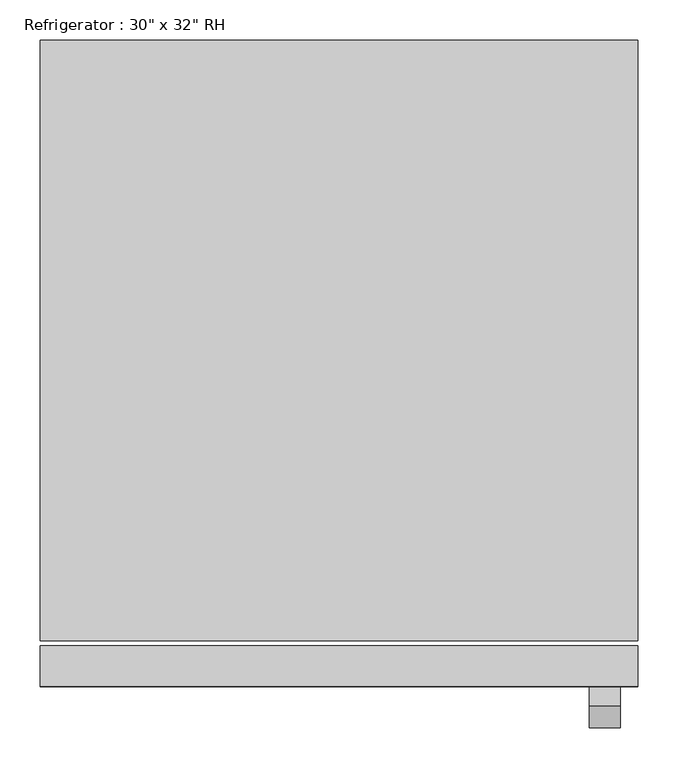
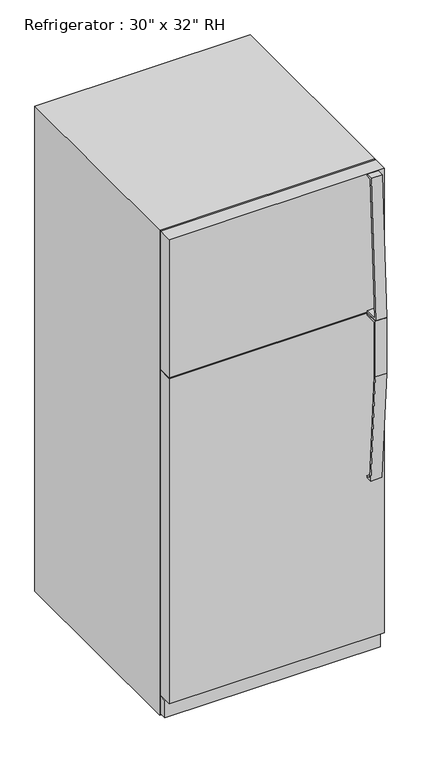
"""IFC4 building model written with IfcOpenShell, lengths in millimetres: proxy geometry."""

import ifcopenshell
import ifcopenshell.guid

model = None  # the IFC model being written
_history = None  # IfcOwnerHistory: only IFC2X3 demands one
_inside = {}  # id of a spatial element -> (the spatial element, [elements in it])
_under = {}  # id of a project, library or spatial element -> (it, [spatial elements below it])
_declared = {}  # id of a project -> (the project, [libraries it declares])
_typed = {}  # id of a type object -> (the type object, [elements of that type])
_made_of = {}  # id of a material, layer set ... -> (it, [elements and type objects made of it])


def new_model(schema):
    """Start an empty IFC model of exactly this schema.

    Asked for "IFC4X3", IfcOpenShell would pick the latest addendum, in which some entities
    have other attributes; the version numbers below select the first issue.
    IFC2X3 requires an IfcOwnerHistory on every rooted entity: one is made here for all.
    """
    global model, _history
    if schema == "IFC4X3":
        model = ifcopenshell.file(schema_version=(4, 3, 0, 0))
    else:
        model = ifcopenshell.file(schema=schema)
    _inside.clear()
    _under.clear()
    _declared.clear()
    _typed.clear()
    _made_of.clear()
    _history = None
    if model.schema == "IFC2X3":
        org = make("IfcOrganization", Name="unknown")
        user = make(
            "IfcPersonAndOrganization",
            ThePerson=make("IfcPerson", FamilyName="unknown"),
            TheOrganization=org,
        )
        app = make(
            "IfcApplication",
            ApplicationDeveloper=org,
            Version="unknown",
            ApplicationFullName="unknown",
            ApplicationIdentifier="unknown",
        )
        _history = make(
            "IfcOwnerHistory",
            OwningUser=user,
            OwningApplication=app,
            ChangeAction="ADDED",
            CreationDate=0,
        )
    return model


def make(cls, **values):
    """One entity of the class cls with the attributes given. An attribute that is None is left unset."""
    return model.create_entity(
        cls, **{name: value for name, value in values.items() if value is not None}
    )


def rooted(cls, **values):
    """An entity with a GlobalId (a new one), such as an element, a storey or a relation."""
    return make(cls, GlobalId=ifcopenshell.guid.new(), OwnerHistory=_history, **values)


def si_unit(unit_type, name, prefix=None):
    """IfcSIUnit, for example si_unit("LENGTHUNIT", "METRE", prefix="MILLI")."""
    return make("IfcSIUnit", UnitType=unit_type, Prefix=prefix, Name=name)


def assignment(units):
    """IfcUnitAssignment: the units of a project."""
    return None if units is None else make("IfcUnitAssignment", Units=units)


def point(xyz):
    """IfcCartesianPoint."""
    return None if xyz is None else make("IfcCartesianPoint", Coordinates=xyz)


def direction(xyz):
    """IfcDirection."""
    return None if xyz is None else make("IfcDirection", DirectionRatios=xyz)


def frame(location, z_axis=None, x_axis=None):
    """IfcAxis2Placement3D, a coordinate frame: its origin and axes. An axis left out is left unset."""
    return make(
        "IfcAxis2Placement3D",
        Location=point(location),
        Axis=direction(z_axis),
        RefDirection=direction(x_axis),
    )


def origin():
    """The frame at (0, 0, 0) with its axes left unset."""
    return frame((0.0, 0.0, 0.0))


def origin_with_axes():
    """The frame at (0, 0, 0) with the z axis (0, 0, 1) and the x axis (1, 0, 0) written out."""
    return frame((0.0, 0.0, 0.0), z_axis=(0.0, 0.0, 1.0), x_axis=(1.0, 0.0, 0.0))


def place(relative_to, where):
    """IfcLocalPlacement: puts the frame where relative to a parent placement (None: the world)."""
    return make(
        "IfcLocalPlacement", PlacementRelTo=relative_to, RelativePlacement=where
    )


def context(
    kind, dimensions, precision=None, world=None, true_north=None, identifier=None
):
    """IfcGeometricRepresentationContext, for example the 3D "Model" context."""
    return make(
        "IfcGeometricRepresentationContext",
        ContextIdentifier=identifier,
        ContextType=kind,
        CoordinateSpaceDimension=dimensions,
        Precision=precision,
        WorldCoordinateSystem=world,
        TrueNorth=true_north,
    )


def project(units=None, contexts=None):
    """IfcProject with its units and contexts."""
    return rooted(
        "IfcProject",
        Name="project",
        RepresentationContexts=contexts,
        UnitsInContext=assignment(units),
    )


def spatial(cls, under=None, at=None, **own):
    """A site, building, storey or space (cls), placed at a placement, below another one or the project."""
    s = rooted(cls, ObjectPlacement=at, **own)
    if under is not None:
        _under.setdefault(under.id(), (under, []))[1].append(s)
    return s


def polyline(points):
    """IfcPolyline through the points."""
    return make("IfcPolyline", Points=[point(p) for p in points])


def outline(outer, holes=None, kind="AREA"):
    """IfcArbitraryClosedProfileDef: a profile drawn as a closed curve; with holes, ...WithVoids."""
    if holes is None:
        return make("IfcArbitraryClosedProfileDef", ProfileType=kind, OuterCurve=outer)
    return make(
        "IfcArbitraryProfileDefWithVoids",
        ProfileType=kind,
        OuterCurve=outer,
        InnerCurves=holes,
    )


def extrude(swept, where, along, depth):
    """IfcExtrudedAreaSolid: the profile swept, set in the frame where, extruded along a direction by depth."""
    return make(
        "IfcExtrudedAreaSolid",
        SweptArea=swept,
        Position=where,
        ExtrudedDirection=direction(along),
        Depth=depth,
    )


def shape(context_of_items, identifier, shape_type, items):
    """IfcShapeRepresentation: the items that make up one representation, for example the "Body"."""
    return make(
        "IfcShapeRepresentation",
        ContextOfItems=context_of_items,
        RepresentationIdentifier=identifier,
        RepresentationType=shape_type,
        Items=items,
    )


def source(mapping_origin, context_of_items, identifier, shape_type, items):
    """IfcRepresentationMap: a shape defined once, which mapped items show again and again."""
    return make(
        "IfcRepresentationMap",
        MappingOrigin=mapping_origin,
        MappedRepresentation=shape(context_of_items, identifier, shape_type, items),
    )


def transform(
    local_origin,
    x_axis=None,
    y_axis=None,
    z_axis=None,
    scale=None,
    scale2=None,
    scale3=None,
    uniform=True,
):
    """IfcCartesianTransformationOperator3D, or its non-uniform kind. x_axis, y_axis, z_axis: its Axis1, 2, 3."""
    if uniform:
        return make(
            "IfcCartesianTransformationOperator3D",
            Axis1=direction(x_axis),
            Axis2=direction(y_axis),
            LocalOrigin=point(local_origin),
            Scale=scale,
            Axis3=direction(z_axis),
        )
    return make(
        "IfcCartesianTransformationOperator3DnonUniform",
        Axis1=direction(x_axis),
        Axis2=direction(y_axis),
        LocalOrigin=point(local_origin),
        Scale=scale,
        Axis3=direction(z_axis),
        Scale2=scale2,
        Scale3=scale3,
    )


def mapped(mapping_source, mapping_target):
    """IfcMappedItem: shows the shape of a source again, moved by a transform."""
    return make(
        "IfcMappedItem", MappingSource=mapping_source, MappingTarget=mapping_target
    )


def made_of(thing, what):
    """Note that an element or type object is made of a material, layer set ...; save() writes the relation."""
    if what is not None:
        _made_of.setdefault(what.id(), (what, []))[1].append(thing)
    return thing


def element(
    cls,
    number,
    at=None,
    inside=None,
    cuts=None,
    type_object=None,
    material=None,
    context=None,
    identifier="Body",
    shape_type=None,
    held_by="IfcProductDefinitionShape",
    body=None,
    shapes=None,
    **own,
):
    """One element of the class cls, such as IfcWall. Its Tag is "e" and its number.

    at: its placement. inside: the storey or other place that contains it. cuts: it is an
    opening in that element (IfcRelVoidsElement). A single representation is given by context,
    identifier, shape_type and body (its items); several are given by shapes. held_by: the class
    of the entity that holds the representations. save() writes the other relations.
    """
    e = rooted(cls, Tag="e%d" % number, ObjectPlacement=at, **own)
    if body is not None:
        shapes = [shape(context, identifier, shape_type, body)]
    if shapes is not None:
        e.Representation = make(held_by, Representations=shapes)
    if inside is not None:
        _inside.setdefault(inside.id(), (inside, []))[1].append(e)
    if cuts is not None:
        rooted(
            "IfcRelVoidsElement", RelatingBuildingElement=cuts, RelatedOpeningElement=e
        )
    if type_object is not None:
        _typed.setdefault(type_object.id(), (type_object, []))[1].append(e)
    return made_of(e, material)


def aggregate(whole, parts):
    """IfcRelAggregates: a whole, such as a stair, and the parts it consists of."""
    return rooted("IfcRelAggregates", RelatingObject=whole, RelatedObjects=parts)


def save(model, path):
    """Write the relations noted so far, then the file.

    IfcRelAggregates (storeys below a building ...), IfcRelContainedInSpatialStructure (elements
    in a storey), IfcRelDefinesByType, IfcRelAssociatesMaterial and IfcRelDeclares: one each for
    every whole, place, type object, material and project.
    """
    for whole, parts in _under.values():
        aggregate(whole, parts)
    for where, things in _inside.values():
        rooted(
            "IfcRelContainedInSpatialStructure",
            RelatedElements=things,
            RelatingStructure=where,
        )
    for kind, things in _typed.values():
        rooted("IfcRelDefinesByType", RelatedObjects=things, RelatingType=kind)
    for what, things in _made_of.values():
        rooted("IfcRelAssociatesMaterial", RelatedObjects=things, RelatingMaterial=what)
    for by, libraries in _declared.values():
        rooted("IfcRelDeclares", RelatingContext=by, RelatedDefinitions=libraries)
    model.write(path)


def proxy_a13a33b2(model_context):
    return source(origin(), model_context, "Body", "SweptSolid", [
        extrude(outline(polyline([(-417.9010285, 1262.0625), (-462.3510285, 1262.0625), (-462.3510285, 1065.4342469), (-434.8723987, 672.4715334), (-417.9010285, 672.4715334), (-417.9010285, 666.1370017), (-440.7949512, 666.1370017), (-468.7010285, 1065.2125), (-468.7010285, 1268.4125), (-417.9010285, 1268.4125), (-417.9010285, 1262.0625)])), frame((312.7375, 0.0, 0.0), z_axis=(1.0, 0.0, 0.0), x_axis=(0.0, 1.0, 0.0)), (0.0, 0.0, 1.0), 38.4332978),
        extrude(outline(polyline([(-442.739413, 1778.0), (-418.6780855, 1778.0), (-418.6780855, 1771.65), (-437.5263449, 1771.65), (-463.4007207, 1277.9375), (-418.6780855, 1277.9375), (-418.6780855, 1271.5875), (-469.2793675, 1271.5875), (-442.739413, 1778.0)])), frame((312.7375, 0.0, 0.0), z_axis=(1.0, 0.0, 0.0), x_axis=(0.0, 1.0, 0.0)), (0.0, 0.0, 1.0), 38.4332978),
        extrude(outline(polyline([(373.0625, -367.1010285), (373.0625, -392.5010285), (-373.0625, -392.5010285), (-373.0625, -367.1010285), (373.0625, -367.1010285)])), frame((0.0, 0.0, 9.3816357), z_axis=(0.0, 0.0, 1.0), x_axis=(1.0, 0.0, 0.0)), (0.0, 0.0, 1.0), 63.5),
        extrude(outline(polyline([(373.0625, -367.1010285), (373.0625, -417.9010285), (-373.0625, -417.9010285), (-373.0625, -367.1010285), (373.0625, -367.1010285)])), frame((0.0, 0.0, 76.2), z_axis=(0.0, 0.0, 1.0), x_axis=(1.0, 0.0, 0.0)), (0.0, 0.0, 1.0), 1192.2125),
        extrude(outline(polyline([(373.0625, -367.1010285), (373.0625, -417.9010285), (-373.0625, -417.9010285), (-373.0625, -367.1010285), (373.0625, -367.1010285)])), frame((0.0, 0.0, 1271.5875), z_axis=(0.0, 0.0, 1.0), x_axis=(1.0, 0.0, 0.0)), (0.0, 0.0, 1.0), 506.4125),
        extrude(outline(polyline([(373.0625, 388.5489715), (373.0625, -360.7510285), (-373.0625, -360.7510285), (-373.0625, 388.5489715), (373.0625, 388.5489715)])), origin_with_axes(), (0.0, 0.0, 1.0), 1778.0),
    ])


if __name__ == "__main__":
    model = new_model("IFC4")
    model_context = context("Model", 3, world=origin())
    ifc_project = project(units=[si_unit("LENGTHUNIT", "METRE", prefix="MILLI")], contexts=[model_context])
    site = spatial("IfcSite", under=ifc_project)
    building = spatial("IfcBuilding", under=site)
    placement = place(None, origin())
    proxy_shape = proxy_a13a33b2(model_context)
    element("IfcBuildingElementProxy", 1, Name="Refrigerator : 30\" x 32\" RH", ObjectType="Refrigerator : 30\" x 32\" RH", at=placement, inside=building, context=model_context, shape_type="MappedRepresentation", body=[
        mapped(proxy_shape, transform((0.0, 0.0, 0.0), x_axis=(1.0, 0.0, 0.0), y_axis=(0.0, 1.0, 0.0), z_axis=(0.0, 0.0, 1.0))),
    ])
    save(model, "model.ifc")

# Revit data of these elements
# Type "Refrigerator : 30\" x 32\" RH"
#   Label = "REF."
#   Assembly Code = "E1090400"
#   Depth = 2' - 7 3/4"
#   Handle = 2' - 3"
#   Height = 5' - 10"
#   Rear Clearance = 0' - 2"
#   Top Door Height = 1' - 8"
#   Width = 2' - 5 3/8"
#   Material = Metal - Paint Finish - Ivory, Glossy
# Element 1 (IfcBuildingElementProxy, "Refrigerator : 30\" x 32\" RH")
#   Materials on its faces: "Metal - Paint Finish - Ivory, Glossy", "Metal - Chrome"
# Materials
#   "Metal - Paint Finish - Ivory, Glossy": class "Paint", colour RGB 247 247 239, transparency 0
#   "Metal - Chrome": class "Metal", colour RGB 17 17 17, transparency 0
